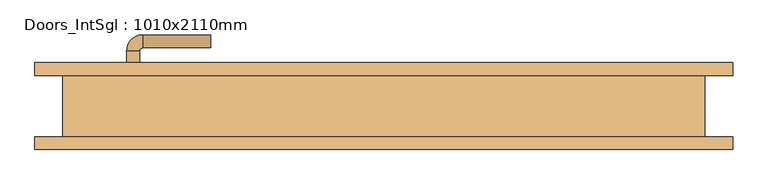
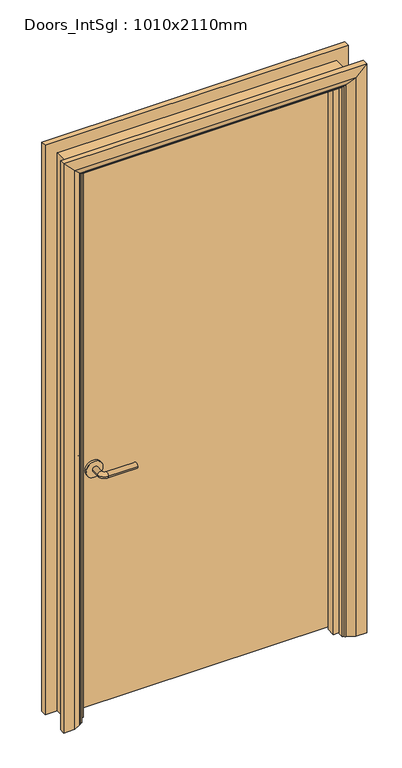
"""IFC4 building model written with IfcOpenShell, lengths in millimetres: door geometry, Doors_IntSgl : 1010x2110mm."""

import ifcopenshell
import ifcopenshell.guid

model = None  # the IFC model being written
_history = None  # IfcOwnerHistory: only IFC2X3 demands one
_inside = {}  # id of a spatial element -> (the spatial element, [elements in it])
_under = {}  # id of a project, library or spatial element -> (it, [spatial elements below it])
_declared = {}  # id of a project -> (the project, [libraries it declares])
_typed = {}  # id of a type object -> (the type object, [elements of that type])
_made_of = {}  # id of a material, layer set ... -> (it, [elements and type objects made of it])


def new_model(schema):
    """Start an empty IFC model of exactly this schema.

    Asked for "IFC4X3", IfcOpenShell would pick the latest addendum, in which some entities
    have other attributes; the version numbers below select the first issue.
    IFC2X3 requires an IfcOwnerHistory on every rooted entity: one is made here for all.
    """
    global model, _history
    if schema == "IFC4X3":
        model = ifcopenshell.file(schema_version=(4, 3, 0, 0))
    else:
        model = ifcopenshell.file(schema=schema)
    _inside.clear()
    _under.clear()
    _declared.clear()
    _typed.clear()
    _made_of.clear()
    _history = None
    if model.schema == "IFC2X3":
        org = make("IfcOrganization", Name="unknown")
        user = make(
            "IfcPersonAndOrganization",
            ThePerson=make("IfcPerson", FamilyName="unknown"),
            TheOrganization=org,
        )
        app = make(
            "IfcApplication",
            ApplicationDeveloper=org,
            Version="unknown",
            ApplicationFullName="unknown",
            ApplicationIdentifier="unknown",
        )
        _history = make(
            "IfcOwnerHistory",
            OwningUser=user,
            OwningApplication=app,
            ChangeAction="ADDED",
            CreationDate=0,
        )
    return model


def make(cls, **values):
    """One entity of the class cls with the attributes given. An attribute that is None is left unset."""
    return model.create_entity(
        cls, **{name: value for name, value in values.items() if value is not None}
    )


def rooted(cls, **values):
    """An entity with a GlobalId (a new one), such as an element, a storey or a relation."""
    return make(cls, GlobalId=ifcopenshell.guid.new(), OwnerHistory=_history, **values)


def si_unit(unit_type, name, prefix=None):
    """IfcSIUnit, for example si_unit("LENGTHUNIT", "METRE", prefix="MILLI")."""
    return make("IfcSIUnit", UnitType=unit_type, Prefix=prefix, Name=name)


def assignment(units):
    """IfcUnitAssignment: the units of a project."""
    return None if units is None else make("IfcUnitAssignment", Units=units)


def point(xyz):
    """IfcCartesianPoint."""
    return None if xyz is None else make("IfcCartesianPoint", Coordinates=xyz)


def direction(xyz):
    """IfcDirection."""
    return None if xyz is None else make("IfcDirection", DirectionRatios=xyz)


def frame(location, z_axis=None, x_axis=None):
    """IfcAxis2Placement3D, a coordinate frame: its origin and axes. An axis left out is left unset."""
    return make(
        "IfcAxis2Placement3D",
        Location=point(location),
        Axis=direction(z_axis),
        RefDirection=direction(x_axis),
    )


def frame_2d(location, x_axis=None):
    """IfcAxis2Placement2D, a coordinate frame in the plane: its origin and x axis."""
    return make(
        "IfcAxis2Placement2D", Location=point(location), RefDirection=direction(x_axis)
    )


def origin():
    """The frame at (0, 0, 0) with its axes left unset."""
    return frame((0.0, 0.0, 0.0))


def place(relative_to, where):
    """IfcLocalPlacement: puts the frame where relative to a parent placement (None: the world)."""
    return make(
        "IfcLocalPlacement", PlacementRelTo=relative_to, RelativePlacement=where
    )


def context(
    kind, dimensions, precision=None, world=None, true_north=None, identifier=None
):
    """IfcGeometricRepresentationContext, for example the 3D "Model" context."""
    return make(
        "IfcGeometricRepresentationContext",
        ContextIdentifier=identifier,
        ContextType=kind,
        CoordinateSpaceDimension=dimensions,
        Precision=precision,
        WorldCoordinateSystem=world,
        TrueNorth=true_north,
    )


def project(units=None, contexts=None):
    """IfcProject with its units and contexts."""
    return rooted(
        "IfcProject",
        Name="project",
        RepresentationContexts=contexts,
        UnitsInContext=assignment(units),
    )


def spatial(cls, under=None, at=None, **own):
    """A site, building, storey or space (cls), placed at a placement, below another one or the project."""
    s = rooted(cls, ObjectPlacement=at, **own)
    if under is not None:
        _under.setdefault(under.id(), (under, []))[1].append(s)
    return s


def polyline(points):
    """IfcPolyline through the points."""
    return make("IfcPolyline", Points=[point(p) for p in points])


def circle_curve(where, radius):
    """IfcCircle in the frame where."""
    return make("IfcCircle", Position=where, Radius=radius)


def ellipse_curve(where, semi_axis1, semi_axis2):
    """IfcEllipse in the frame where."""
    return make(
        "IfcEllipse", Position=where, SemiAxis1=semi_axis1, SemiAxis2=semi_axis2
    )


def trimmed(basis, trim1, trim2, sense, master):
    """IfcTrimmedCurve: the piece of a basis curve between two trims."""
    return make(
        "IfcTrimmedCurve",
        BasisCurve=basis,
        Trim1=trim1,
        Trim2=trim2,
        SenseAgreement=sense,
        MasterRepresentation=master,
    )


def segment(curve, same_sense, transition):
    """IfcCompositeCurveSegment."""
    return make(
        "IfcCompositeCurveSegment",
        Transition=transition,
        SameSense=same_sense,
        ParentCurve=curve,
    )


def composite_curve(segments, self_intersect=None):
    """IfcCompositeCurve: segments joined end to end."""
    return make("IfcCompositeCurve", Segments=segments, SelfIntersect=self_intersect)


def outline(outer, holes=None, kind="AREA"):
    """IfcArbitraryClosedProfileDef: a profile drawn as a closed curve; with holes, ...WithVoids."""
    if holes is None:
        return make("IfcArbitraryClosedProfileDef", ProfileType=kind, OuterCurve=outer)
    return make(
        "IfcArbitraryProfileDefWithVoids",
        ProfileType=kind,
        OuterCurve=outer,
        InnerCurves=holes,
    )


def extrude(swept, where, along, depth):
    """IfcExtrudedAreaSolid: the profile swept, set in the frame where, extruded along a direction by depth."""
    return make(
        "IfcExtrudedAreaSolid",
        SweptArea=swept,
        Position=where,
        ExtrudedDirection=direction(along),
        Depth=depth,
    )


def faces_of(points, faces, orient=None, outer=None):
    """IfcFace entities. A face is a list of loops; a loop is a list of indices into points, from 0.

    orient and outer hold one flag for each loop. By default every Orientation is true, the
    first loop of a face is its IfcFaceOuterBound and the others are IfcFaceBound.
    """
    made = []
    for i, loops in enumerate(faces):
        bounds = []
        for j, loop in enumerate(loops):
            is_outer = j == 0 if outer is None else outer[i][j]
            bounds.append(
                make(
                    "IfcFaceOuterBound" if is_outer else "IfcFaceBound",
                    Bound=make("IfcPolyLoop", Polygon=[points[k] for k in loop]),
                    Orientation=True if orient is None else orient[i][j],
                )
            )
        made.append(make("IfcFace", Bounds=bounds))
    return made


def faceted_brep(points, faces, orient=None, outer=None, voids=None):
    """IfcFacetedBrep: a solid bounded by flat faces; with voids (closed shells), ...WithVoids."""
    shared = [point(p) for p in points]
    hull = make("IfcClosedShell", CfsFaces=faces_of(shared, faces, orient, outer))
    if voids is None:
        return make("IfcFacetedBrep", Outer=hull)
    return make(
        "IfcFacetedBrepWithVoids",
        Outer=hull,
        Voids=[
            make(cls, CfsFaces=faces_of(shared, fs, o, b)) for cls, fs, o, b in voids
        ],
    )


def shape(context_of_items, identifier, shape_type, items):
    """IfcShapeRepresentation: the items that make up one representation, for example the "Body"."""
    return make(
        "IfcShapeRepresentation",
        ContextOfItems=context_of_items,
        RepresentationIdentifier=identifier,
        RepresentationType=shape_type,
        Items=items,
    )


def source(mapping_origin, context_of_items, identifier, shape_type, items):
    """IfcRepresentationMap: a shape defined once, which mapped items show again and again."""
    return make(
        "IfcRepresentationMap",
        MappingOrigin=mapping_origin,
        MappedRepresentation=shape(context_of_items, identifier, shape_type, items),
    )


def transform(
    local_origin,
    x_axis=None,
    y_axis=None,
    z_axis=None,
    scale=None,
    scale2=None,
    scale3=None,
    uniform=True,
):
    """IfcCartesianTransformationOperator3D, or its non-uniform kind. x_axis, y_axis, z_axis: its Axis1, 2, 3."""
    if uniform:
        return make(
            "IfcCartesianTransformationOperator3D",
            Axis1=direction(x_axis),
            Axis2=direction(y_axis),
            LocalOrigin=point(local_origin),
            Scale=scale,
            Axis3=direction(z_axis),
        )
    return make(
        "IfcCartesianTransformationOperator3DnonUniform",
        Axis1=direction(x_axis),
        Axis2=direction(y_axis),
        LocalOrigin=point(local_origin),
        Scale=scale,
        Axis3=direction(z_axis),
        Scale2=scale2,
        Scale3=scale3,
    )


def mapped(mapping_source, mapping_target):
    """IfcMappedItem: shows the shape of a source again, moved by a transform."""
    return make(
        "IfcMappedItem", MappingSource=mapping_source, MappingTarget=mapping_target
    )


def made_of(thing, what):
    """Note that an element or type object is made of a material, layer set ...; save() writes the relation."""
    if what is not None:
        _made_of.setdefault(what.id(), (what, []))[1].append(thing)
    return thing


def element(
    cls,
    number,
    at=None,
    inside=None,
    cuts=None,
    type_object=None,
    material=None,
    context=None,
    identifier="Body",
    shape_type=None,
    held_by="IfcProductDefinitionShape",
    body=None,
    shapes=None,
    **own,
):
    """One element of the class cls, such as IfcWall. Its Tag is "e" and its number.

    at: its placement. inside: the storey or other place that contains it. cuts: it is an
    opening in that element (IfcRelVoidsElement). A single representation is given by context,
    identifier, shape_type and body (its items); several are given by shapes. held_by: the class
    of the entity that holds the representations. save() writes the other relations.
    """
    e = rooted(cls, Tag="e%d" % number, ObjectPlacement=at, **own)
    if body is not None:
        shapes = [shape(context, identifier, shape_type, body)]
    if shapes is not None:
        e.Representation = make(held_by, Representations=shapes)
    if inside is not None:
        _inside.setdefault(inside.id(), (inside, []))[1].append(e)
    if cuts is not None:
        rooted(
            "IfcRelVoidsElement", RelatingBuildingElement=cuts, RelatedOpeningElement=e
        )
    if type_object is not None:
        _typed.setdefault(type_object.id(), (type_object, []))[1].append(e)
    return made_of(e, material)


def aggregate(whole, parts):
    """IfcRelAggregates: a whole, such as a stair, and the parts it consists of."""
    return rooted("IfcRelAggregates", RelatingObject=whole, RelatedObjects=parts)


def save(model, path):
    """Write the relations noted so far, then the file.

    IfcRelAggregates (storeys below a building ...), IfcRelContainedInSpatialStructure (elements
    in a storey), IfcRelDefinesByType, IfcRelAssociatesMaterial and IfcRelDeclares: one each for
    every whole, place, type object, material and project.
    """
    for whole, parts in _under.values():
        aggregate(whole, parts)
    for where, things in _inside.values():
        rooted(
            "IfcRelContainedInSpatialStructure",
            RelatedElements=things,
            RelatingStructure=where,
        )
    for kind, things in _typed.values():
        rooted("IfcRelDefinesByType", RelatedObjects=things, RelatingType=kind)
    for what, things in _made_of.values():
        rooted("IfcRelAssociatesMaterial", RelatedObjects=things, RelatingMaterial=what)
    for by, libraries in _declared.values():
        rooted("IfcRelDeclares", RelatingContext=by, RelatedDefinitions=libraries)
    model.write(path)


def plane_surface(at):
    """IfcPlane: the flat surface through the origin of the frame at, square to its z axis."""
    return make("IfcPlane", Position=at)


def cylinder_surface(at, radius):
    """IfcCylindricalSurface: all points at the distance radius from the z axis of the frame at."""
    return make("IfcCylindricalSurface", Position=at, Radius=radius)


def revolved_surface(curve, axis_point, axis_direction):
    """IfcSurfaceOfRevolution: the curve turned about the line through axis_point along axis_direction."""
    return make(
        "IfcSurfaceOfRevolution",
        SweptCurve=make("IfcArbitraryOpenProfileDef", ProfileType="CURVE", Curve=curve),
        AxisPosition=make("IfcAxis1Placement", Location=point(axis_point), Axis=direction(axis_direction)),
    )


def advanced_brep(points, edges, surfaces, faces):
    """IfcAdvancedBrep: a solid bounded by faces that lie on surfaces and meet in shared edges.

    An edge is (start, end): straight between two places in points (the first is 0);
    or (start, end, curve); or (start, end, curve, False) where it runs against its curve.
    A face is (place in surfaces, loops), or (place, loops, False) where it looks against
    its surface's normal. A loop lists edges by number (the first is 1), with a minus sign
    where the edge is run from its end to its start. The first loop is the outer one.
    """
    corners = [point(p) for p in points]
    vertices = [make("IfcVertexPoint", VertexGeometry=c) for c in corners]
    made = []
    for start, end, *more in edges:
        made.append(
            make(
                "IfcEdgeCurve",
                EdgeStart=vertices[start],
                EdgeEnd=vertices[end],
                EdgeGeometry=more[0] if more else make("IfcPolyline", Points=[corners[start], corners[end]]),
                SameSense=more[1] if len(more) > 1 else True,
            )
        )
    hull = []
    for where, loops, *sense in faces:
        bounds = []
        for j, loop in enumerate(loops):
            ring = [make("IfcOrientedEdge", EdgeElement=made[abs(k) - 1], Orientation=k > 0) for k in loop]
            bounds.append(
                make(
                    "IfcFaceOuterBound" if j == 0 else "IfcFaceBound",
                    Bound=make("IfcEdgeLoop", EdgeList=ring),
                    Orientation=True,
                )
            )
        hull.append(make("IfcAdvancedFace", Bounds=bounds, FaceSurface=surfaces[where], SameSense=sense[0] if sense else True))
    return make("IfcAdvancedBrep", Outer=make("IfcClosedShell", CfsFaces=hull))


def doors_intsgl_1010x2110mm_9b3ab836(model_context):
    return source(origin(), model_context, "Body", "SolidModel", [
        advanced_brep(
        [(-398.0, 1.5, 900.0), (-378.0, 1.5, 900.0), (-378.0, -28.5, 900.0), (-398.0, -28.5, 900.0), (-373.0, -33.5, 900.0), (-373.0, -53.5, 900.0), (-268.0, -53.5, 900.0), (-268.0, -33.5, 900.0)],
        [
            (0, 1, circle_curve(frame((-388.0, 1.5, 900.0), z_axis=(0.0, 1.0, 0.0), x_axis=(1.0, 0.0, 0.0)), 10.0)),
            (1, 0, circle_curve(frame((-388.0, 1.5, 900.0), z_axis=(0.0, 1.0, 0.0), x_axis=(1.0, 0.0, 0.0)), 10.0)),
            (1, 2),
            (2, 3, circle_curve(frame((-388.0, -28.5, 900.0), z_axis=(0.0, 1.0, 0.0), x_axis=(1.0, 0.0, 0.0)), 10.0)),
            (3, 0),
            (3, 2, circle_curve(frame((-388.0, -28.5, 900.0), z_axis=(0.0, 1.0, 0.0), x_axis=(1.0, 0.0, 0.0)), 10.0)),
            (4, 5, circle_curve(frame((-373.0, -43.5, 900.0), z_axis=(-1.0, 0.0, 0.0), x_axis=(0.0, 1.0, 0.0)), 10.0)),
            (5, 3, circle_curve(frame((-373.0, -28.5, 900.0), z_axis=(0.0, 0.0, -1.0), x_axis=(-1.0, 0.0, 0.0)), 25.0)),
            (2, 4, circle_curve(frame((-373.0, -28.5, 900.0), z_axis=(0.0, 0.0, 1.0), x_axis=(-1.0, 0.0, 0.0)), 5.0)),
            (5, 4, circle_curve(frame((-373.0, -43.5, 900.0), z_axis=(-1.0, 0.0, 0.0), x_axis=(0.0, 1.0, 0.0)), 10.0)),
            (6, 7, circle_curve(frame((-268.0, -43.5, 900.0), z_axis=(1.0, 0.0, 0.0), x_axis=(0.0, 1.0, 0.0)), 10.0)),
            (7, 6, circle_curve(frame((-268.0, -43.5, 900.0), z_axis=(1.0, 0.0, 0.0), x_axis=(0.0, 1.0, 0.0)), 10.0)),
            (4, 7),
            (6, 5),
        ],
        [
            plane_surface(frame((-388.0, 1.5, 900.0), z_axis=(0.0, 1.0, 0.0), x_axis=(0.0, 0.0, 1.0))),
            cylinder_surface(frame((-388.0, 1.5, 900.0), z_axis=(0.0, 1.0, 0.0), x_axis=(1.0, 0.0, 0.0)), 10.0),
            revolved_surface(trimmed(ellipse_curve(frame((-388.0, -28.5, 900.0), z_axis=(0.0, -1.0, 0.0), x_axis=(1.0, 0.0, 0.0)), 10.0, 10.0), [point((-398.0, -28.5, 900.0))], [point((-378.0, -28.5, 900.0))], True, "CARTESIAN"), (-373.0, -28.5, 900.0), (0.0, 0.0, -1.0)),
            revolved_surface(trimmed(ellipse_curve(frame((-388.0, -28.5, 900.0), z_axis=(0.0, -1.0, 0.0), x_axis=(1.0, 0.0, 0.0)), 10.0, 10.0), [point((-378.0, -28.5, 900.0))], [point((-398.0, -28.5, 900.0))], True, "CARTESIAN"), (-373.0, -28.5, 900.0), (0.0, 0.0, -1.0)),
            plane_surface(frame((-268.0, -43.5, 900.0), z_axis=(1.0, 0.0, 0.0), x_axis=(0.0, 0.0, 1.0))),
            cylinder_surface(frame((-373.0, -43.5, 900.0), z_axis=(-1.0, 0.0, 0.0), x_axis=(0.0, 1.0, 0.0)), 10.0),
        ],
        [
            (0, [[1, 2]]),
            (1, [[3, 4, 5, -2]]),
            (1, [[-5, 6, -3, -1]]),
            (2, [[7, 8, -4, 9]]),
            (3, [[10, -9, -6, -8]]),
            (4, [[11, 12]]),
            (5, [[13, -11, 14, -7]]),
            (5, [[-14, -12, -13, -10]]),
        ],
    ),
        extrude(outline(composite_curve([segment(trimmed(circle_curve(frame_2d((900.0, -390.5)), 30.0), [point((900.0, -420.5))], [point((900.0, -360.5))], False, "CARTESIAN"), True, "CONTINUOUS"), segment(trimmed(circle_curve(frame_2d((900.0, -390.5)), 30.0), [point((900.0, -360.5))], [point((900.0, -420.5))], False, "CARTESIAN"), True, "CONTINUOUS")], self_intersect=False)), frame((0.0, 1.5, 0.0), z_axis=(0.0, 1.0, 0.0), x_axis=(0.0, 0.0, 1.0)), (0.0, 0.0, 1.0), 8.0),
        advanced_brep(
        [(-398.0, 55.5, 900.0), (-378.0, 55.5, 900.0), (-398.0, 85.5, 900.0), (-378.0, 85.5, 900.0), (-373.0, 90.5, 900.0), (-373.0, 110.5, 900.0), (-268.0, 110.5, 900.0), (-268.0, 90.5, 900.0)],
        [
            (0, 1, circle_curve(frame((-388.0, 55.5, 900.0), z_axis=(0.0, -1.0, 0.0), x_axis=(1.0, 0.0, 0.0)), 10.0)),
            (1, 0, circle_curve(frame((-388.0, 55.5, 900.0), z_axis=(0.0, -1.0, 0.0), x_axis=(1.0, 0.0, 0.0)), 10.0)),
            (0, 2),
            (2, 3, circle_curve(frame((-388.0, 85.5, 900.0), z_axis=(0.0, -1.0, 0.0), x_axis=(1.0, 0.0, 0.0)), 10.0)),
            (3, 1),
            (3, 2, circle_curve(frame((-388.0, 85.5, 900.0), z_axis=(0.0, -1.0, 0.0), x_axis=(1.0, 0.0, 0.0)), 10.0)),
            (4, 3, circle_curve(frame((-373.0, 85.5, 900.0), z_axis=(0.0, 0.0, 1.0), x_axis=(-1.0, 0.0, 0.0)), 5.0)),
            (2, 5, circle_curve(frame((-373.0, 85.5, 900.0), z_axis=(0.0, 0.0, -1.0), x_axis=(-1.0, 0.0, 0.0)), 25.0)),
            (5, 4, circle_curve(frame((-373.0, 100.5, 900.0), z_axis=(-1.0, 0.0, 0.0), x_axis=(0.0, -1.0, 0.0)), 10.0)),
            (4, 5, circle_curve(frame((-373.0, 100.5, 900.0), z_axis=(-1.0, 0.0, 0.0), x_axis=(0.0, -1.0, 0.0)), 10.0)),
            (6, 7, circle_curve(frame((-268.0, 100.5, 900.0), z_axis=(1.0, 0.0, 0.0), x_axis=(0.0, -1.0, 0.0)), 10.0)),
            (7, 6, circle_curve(frame((-268.0, 100.5, 900.0), z_axis=(1.0, 0.0, 0.0), x_axis=(0.0, -1.0, 0.0)), 10.0)),
            (5, 6),
            (7, 4),
        ],
        [
            plane_surface(frame((-388.0, 55.5, 900.0), z_axis=(0.0, -1.0, 0.0), x_axis=(0.0, 0.0, 1.0))),
            cylinder_surface(frame((-388.0, 55.5, 900.0), z_axis=(0.0, -1.0, 0.0), x_axis=(1.0, 0.0, 0.0)), 10.0),
            revolved_surface(trimmed(ellipse_curve(frame((-388.0, 85.5, 900.0), z_axis=(0.0, -1.0, 0.0), x_axis=(1.0, 0.0, 0.0)), 10.0, 10.0), [point((-398.0, 85.5, 900.0))], [point((-378.0, 85.5, 900.0))], True, "CARTESIAN"), (-373.0, 85.5, 900.0), (0.0, 0.0, -1.0)),
            revolved_surface(trimmed(ellipse_curve(frame((-388.0, 85.5, 900.0), z_axis=(0.0, -1.0, 0.0), x_axis=(1.0, 0.0, 0.0)), 10.0, 10.0), [point((-378.0, 85.5, 900.0))], [point((-398.0, 85.5, 900.0))], True, "CARTESIAN"), (-373.0, 85.5, 900.0), (0.0, 0.0, -1.0)),
            plane_surface(frame((-268.0, 100.5, 900.0), z_axis=(1.0, 0.0, 0.0), x_axis=(0.0, 0.0, 1.0))),
            cylinder_surface(frame((-373.0, 100.5, 900.0), z_axis=(-1.0, 0.0, 0.0), x_axis=(0.0, -1.0, 0.0)), 10.0),
        ],
        [
            (0, [[1, 2]]),
            (1, [[-1, 3, 4, 5]]),
            (1, [[-2, -5, 6, -3]]),
            (2, [[7, -4, 8, 9]]),
            (3, [[-8, -6, -7, 10]]),
            (4, [[11, 12]]),
            (5, [[-9, 13, -12, 14]]),
            (5, [[-10, -14, -11, -13]]),
        ],
    ),
        extrude(outline(composite_curve([segment(trimmed(circle_curve(frame_2d((900.0, -390.5)), 30.0), [point((900.0, -420.5))], [point((900.0, -360.5))], False, "CARTESIAN"), True, "CONTINUOUS"), segment(trimmed(circle_curve(frame_2d((900.0, -390.5)), 30.0), [point((900.0, -360.5))], [point((900.0, -420.5))], False, "CARTESIAN"), True, "CONTINUOUS")], self_intersect=False)), frame((0.0, 47.5, 0.0), z_axis=(0.0, 1.0, 0.0), x_axis=(0.0, 0.0, 1.0)), (0.0, 0.0, 1.0), 8.0),
        extrude(outline(polyline([(463.0, 9.5), (-463.0, 9.5), (-463.0, 47.5), (463.0, 47.5), (463.0, 9.5)])), frame((0.0, 0.0, 8.0), z_axis=(0.0, 0.0, 1.0), x_axis=(1.0, 0.0, 0.0)), (0.0, 0.0, 1.0), 2060.0),
        advanced_brep(
        [(540.0, 67.5, 0.0), (540.0, 47.5, 0.0), (470.0, 47.5, 0.0), (474.0, 53.5, 0.0), (500.0, 67.5, 0.0), (540.0, 67.5, 2145.0), (540.0, 47.5, 2145.0), (-540.0, 47.5, 2145.0), (-540.0, 47.5, 0.0), (-470.0, 47.5, 0.0), (-470.0, 47.5, 2075.0), (470.0, 47.5, 2075.0), (474.0, 53.5, 2079.0), (500.0, 67.5, 2105.0), (-500.0, 67.5, 2105.0), (-500.0, 67.5, 0.0), (-540.0, 67.5, 0.0), (-540.0, 67.5, 2145.0), (-474.0, 53.5, 2079.0), (-474.0, 53.5, 0.0)],
        [
            (0, 1),
            (1, 2),
            (2, 3, circle_curve(frame((478.0, 46.5, 0.0), z_axis=(0.0, 0.0, -1.0), x_axis=(1.0, 0.0, 0.0)), 8.0622577)),
            (3, 4),
            (4, 0),
            (0, 5),
            (5, 6),
            (6, 1),
            (6, 7),
            (7, 8),
            (8, 9),
            (9, 10),
            (10, 11),
            (11, 2),
            (11, 12, ellipse_curve(frame((478.0, 46.5, 2083.0), z_axis=(0.7071067811865475, 0.0, -0.7071067811865475), x_axis=(-0.7071067811865474, 0.0, -0.7071067811865476)), 11.4017543, 8.0622577)),
            (12, 3),
            (12, 13),
            (13, 4),
            (13, 14),
            (14, 15),
            (15, 16),
            (16, 17),
            (17, 5),
            (17, 7),
            (10, 18, ellipse_curve(frame((-478.0, 46.5, 2083.0), z_axis=(0.7071067811865475, 0.0, 0.7071067811865475), x_axis=(0.7071067811865476, 0.0, -0.7071067811865474)), 11.4017543, 8.0622577)),
            (18, 12),
            (18, 14),
            (15, 19),
            (19, 9, circle_curve(frame((-478.0, 46.5, 0.0), z_axis=(0.0, 0.0, -1.0), x_axis=(-1.0, 0.0, 0.0)), 8.0622577)),
            (8, 16),
            (19, 18),
        ],
        [
            plane_surface(frame((470.0, 47.5, 0.0), z_axis=(0.0, 0.0, -1.0), x_axis=(0.0, -1.0, 0.0))),
            plane_surface(frame((540.0, 67.5, 0.0), z_axis=(1.0, 0.0, 0.0), x_axis=(0.0, 0.0, 1.0))),
            plane_surface(frame((540.0, 47.5, 0.0), z_axis=(0.0, -1.0, 0.0), x_axis=(0.0, 0.0, 1.0))),
            cylinder_surface(frame((478.0, 46.5, 0.0), z_axis=(0.0, 0.0, -1.0), x_axis=(1.0, 0.0, 0.0)), 8.0622577),
            plane_surface(frame((474.0, 53.5, 0.0), z_axis=(-0.4740998230350126, 0.880471099922178, 0.0), x_axis=(0.0, 0.0, 1.0))),
            plane_surface(frame((500.0, 67.5, 0.0), z_axis=(0.0, 1.0, 0.0), x_axis=(0.0, 0.0, 1.0))),
            plane_surface(frame((540.0, 67.5, 2145.0), z_axis=(0.0, 0.0, 1.0), x_axis=(-1.0, 0.0, 0.0))),
            cylinder_surface(frame((470.0, 46.5, 2083.0), z_axis=(1.0, 0.0, 0.0), x_axis=(0.0, 0.0, 1.0)), 8.0622577),
            plane_surface(frame((474.0, 53.5, 2079.0), z_axis=(0.0, 0.8804710999221764, -0.4740998230350154), x_axis=(-1.0, 0.0, 0.0))),
            plane_surface(frame((-470.0, 47.5, 0.0), z_axis=(0.0, 0.0, -1.0), x_axis=(0.0, -1.0, 0.0))),
            plane_surface(frame((-540.0, 67.5, 2145.0), z_axis=(-1.0, 0.0, 0.0), x_axis=(0.0, 0.0, -1.0))),
            cylinder_surface(frame((-478.0, 46.5, 2075.0), z_axis=(0.0, 0.0, 1.0), x_axis=(-1.0, 0.0, 0.0)), 8.0622577),
            plane_surface(frame((-474.0, 53.5, 2079.0), z_axis=(0.47409982303501824, 0.8804710999221749, 0.0), x_axis=(0.0, 0.0, -1.0))),
        ],
        [
            (0, [[1, 2, 3, 4, 5]]),
            (1, [[-1, 6, 7, 8]]),
            (2, [[-2, -8, 9, 10, 11, 12, 13, 14]]),
            (3, [[-3, -14, 15, 16]]),
            (4, [[-4, -16, 17, 18]]),
            (5, [[-5, -18, 19, 20, 21, 22, 23, -6]]),
            (6, [[-7, -23, 24, -9]]),
            (7, [[-15, -13, 25, 26]]),
            (8, [[-17, -26, 27, -19]]),
            (9, [[-21, 28, 29, -11, 30]]),
            (10, [[-24, -22, -30, -10]]),
            (11, [[-25, -12, -29, 31]]),
            (12, [[-27, -31, -28, -20]]),
        ],
    ),
        extrude(outline(polyline([(0.0, -465.0), (0.0, -446.0), (2051.0, -446.0), (2051.0, 446.0), (0.0, 446.0), (0.0, 465.0), (2070.0, 465.0), (2070.0, -465.0), (0.0, -465.0)])), frame((0.0, -24.5, 0.0), z_axis=(0.0, 1.0, 0.0), x_axis=(0.0, 0.0, 1.0)), (0.0, 0.0, 1.0), 32.0),
        advanced_brep(
        [(-540.0, -67.5, 0.0), (-540.0, -47.5, 0.0), (-470.0, -47.5, 0.0), (-474.0, -53.5, 0.0), (-500.0, -67.5, 0.0), (-540.0, -67.5, 2145.0), (-540.0, -47.5, 2145.0), (-470.0, -47.5, 2075.0), (-474.0, -53.5, 2079.0), (-500.0, -67.5, 2105.0), (540.0, -67.5, 2145.0), (540.0, -47.5, 2145.0), (470.0, -47.5, 2075.0), (474.0, -53.5, 2079.0), (500.0, -67.5, 2105.0), (540.0, -67.5, 0.0), (500.0, -67.5, 0.0), (474.0, -53.5, 0.0), (470.0, -47.5, 0.0), (540.0, -47.5, 0.0)],
        [
            (0, 1),
            (1, 2),
            (2, 3, circle_curve(frame((-478.0, -46.5, 0.0), z_axis=(0.0, 0.0, -1.0), x_axis=(-1.0, 0.0, 0.0)), 8.0622577)),
            (3, 4),
            (4, 0),
            (0, 5),
            (5, 6),
            (6, 1),
            (6, 7),
            (7, 2),
            (7, 8, ellipse_curve(frame((-478.0, -46.5, 2083.0), z_axis=(-0.7071067811865475, 0.0, -0.7071067811865475), x_axis=(0.7071067811865474, 0.0, -0.7071067811865476)), 11.4017543, 8.0622577)),
            (8, 3),
            (8, 9),
            (9, 4),
            (9, 5),
            (5, 10),
            (10, 11),
            (11, 6),
            (11, 12),
            (12, 7),
            (12, 13, ellipse_curve(frame((478.0, -46.5, 2083.0), z_axis=(-0.7071067811865475, 0.0, 0.7071067811865475), x_axis=(-0.7071067811865476, 0.0, -0.7071067811865474)), 11.4017543, 8.0622577)),
            (13, 8),
            (13, 14),
            (14, 9),
            (14, 10),
            (15, 16),
            (16, 17),
            (17, 18, circle_curve(frame((478.0, -46.5, 0.0), z_axis=(0.0, 0.0, -1.0), x_axis=(1.0, 0.0, 0.0)), 8.0622577)),
            (18, 19),
            (19, 15),
            (10, 15),
            (19, 11),
            (18, 12),
            (17, 13),
            (16, 14),
        ],
        [
            plane_surface(frame((-470.0, -120.3010989, 0.0), z_axis=(0.0, 0.0, -1.0), x_axis=(1.0, 0.0, 0.0))),
            plane_surface(frame((-540.0, -67.5, 0.0), z_axis=(-1.0, 0.0, 0.0), x_axis=(0.0, 0.0, 1.0))),
            plane_surface(frame((-540.0, -47.5, 0.0), z_axis=(0.0, 1.0, 0.0), x_axis=(0.0, 0.0, 1.0))),
            cylinder_surface(frame((-478.0, -46.5, 0.0), z_axis=(0.0, 0.0, -1.0), x_axis=(-1.0, 0.0, 0.0)), 8.0622577),
            plane_surface(frame((-474.0, -53.5, 0.0), z_axis=(0.4740998230350183, -0.8804710999221749, 0.0), x_axis=(0.0, 0.0, 1.0))),
            plane_surface(frame((-500.0, -67.5, 0.0), z_axis=(0.0, -1.0, 0.0), x_axis=(0.0, 0.0, 1.0))),
            plane_surface(frame((-540.0, -67.5, 2145.0), z_axis=(0.0, 0.0, 1.0), x_axis=(1.0, 0.0, 0.0))),
            plane_surface(frame((-540.0, -47.5, 2145.0), z_axis=(0.0, 1.0, 0.0), x_axis=(1.0, 0.0, 0.0))),
            cylinder_surface(frame((-470.0, -46.5, 2083.0), z_axis=(-1.0, 0.0, 0.0), x_axis=(0.0, 0.0, 1.0)), 8.0622577),
            plane_surface(frame((-474.0, -53.5, 2079.0), z_axis=(0.0, -0.8804710999221749, -0.4740998230350183), x_axis=(1.0, 0.0, 0.0))),
            plane_surface(frame((-500.0, -67.5, 2105.0), z_axis=(0.0, -1.0, 0.0), x_axis=(1.0, 0.0, 0.0))),
            plane_surface(frame((470.0, -120.3010989, 0.0), z_axis=(0.0, 0.0, -1.0), x_axis=(-1.0, 0.0, 0.0))),
            plane_surface(frame((540.0, -67.5, 2145.0), z_axis=(1.0, 0.0, 0.0), x_axis=(0.0, 0.0, -1.0))),
            plane_surface(frame((540.0, -47.5, 2145.0), z_axis=(0.0, 1.0, 0.0), x_axis=(0.0, 0.0, -1.0))),
            cylinder_surface(frame((478.0, -46.5, 2075.0), z_axis=(0.0, 0.0, 1.0), x_axis=(1.0, 0.0, 0.0)), 8.0622577),
            plane_surface(frame((474.0, -53.5, 2079.0), z_axis=(-0.4740998230350183, -0.8804710999221749, 0.0), x_axis=(0.0, 0.0, -1.0))),
            plane_surface(frame((500.0, -67.5, 2105.0), z_axis=(0.0, -1.0, 0.0), x_axis=(0.0, 0.0, -1.0))),
        ],
        [
            (0, [[1, 2, 3, 4, 5]]),
            (1, [[-1, 6, 7, 8]]),
            (2, [[-2, -8, 9, 10]]),
            (3, [[-3, -10, 11, 12]]),
            (4, [[-4, -12, 13, 14]]),
            (5, [[-5, -14, 15, -6]]),
            (6, [[-7, 16, 17, 18]]),
            (7, [[-9, -18, 19, 20]]),
            (8, [[-11, -20, 21, 22]]),
            (9, [[-13, -22, 23, 24]]),
            (10, [[-15, -24, 25, -16]]),
            (11, [[26, 27, 28, 29, 30]]),
            (12, [[-17, 31, -30, 32]]),
            (13, [[-19, -32, -29, 33]]),
            (14, [[-21, -33, -28, 34]]),
            (15, [[-23, -34, -27, 35]]),
            (16, [[-25, -35, -26, -31]]),
        ],
    ),
        faceted_brep([(-465.0, 47.5, 0.0), (-465.0, -47.5, 0.0), (-497.0, -47.5, 0.0), (-497.0, 47.5, 0.0), (-465.0, 47.5, 2070.0), (-465.0, -47.5, 2070.0), (-497.0, -47.5, 2102.0), (-497.0, 47.5, 2102.0), (465.0, 47.5, 2070.0), (465.0, -47.5, 2070.0), (497.0, -47.5, 2102.0), (497.0, 47.5, 2102.0), (465.0, 47.5, 0.0), (497.0, 47.5, 0.0), (497.0, -47.5, 0.0), (465.0, -47.5, 0.0)], [[[0, 1, 2, 3]], [[1, 0, 4, 5]], [[2, 1, 5, 6]], [[3, 2, 6, 7]], [[0, 3, 7, 4]], [[5, 4, 8, 9]], [[6, 5, 9, 10]], [[7, 6, 10, 11]], [[4, 7, 11, 8]], [[12, 13, 14, 15]], [[9, 8, 12, 15]], [[10, 9, 15, 14]], [[11, 10, 14, 13]], [[8, 11, 13, 12]]]),
    ])


if __name__ == "__main__":
    model = new_model("IFC4")
    model_context = context("Model", 3, world=origin())
    ifc_project = project(units=[si_unit("LENGTHUNIT", "METRE", prefix="MILLI")], contexts=[model_context])
    site = spatial("IfcSite", under=ifc_project)
    building = spatial("IfcBuilding", under=site)
    placement = place(None, origin())
    doors_intsgl_1010x2110mm_shape = doors_intsgl_1010x2110mm_9b3ab836(model_context)
    element("IfcDoor", 1, ObjectType="Doors_IntSgl : 1010x2110mm", at=placement, inside=building, context=model_context, shape_type="MappedRepresentation", body=[
        mapped(doors_intsgl_1010x2110mm_shape, transform((0.0, 0.0, 0.0), x_axis=(1.0, 0.0, 0.0), y_axis=(0.0, 1.0, 0.0), z_axis=(0.0, 0.0, 1.0))),
    ])
    save(model, "model.ifc")

# Revit data of these elements
# Type "Doors_IntSgl : 1010x2110mm"
#   Construction Type Id = "MDOOR"
#   Type Mark = "43"
#   Type Comments = "Internal Single"
#   Operation = "SingleSwingRight"
#   Manufacturer = "Revit"
#   Keynote = "L20"
#   Description = "Internal Single Door"
#   Analytic Construction = "Metal"
#   UnderCut = 8 mm
#   Tolerance = 2 mm
#   Thickness = 38 mm
#   Thermal Resistance (R) = 0.270117 (m²·K)/W
#   Structural Tolerance = 8 mm
#   StopDepth = 32 mm
#   Stop Thickness = 19 mm
#   Rough Width = 1010 mm
#   Rough Height = 2110 mm
#   Height to Top Lock Rail = 1000 mm
#   Heat Transfer Coefficient (U) = 3.7021 W/(m²·K)
#   Handle Z Distance = 900 mm
#   Handle X Distance = 75 mm
#   Frame Thickness = 32 mm
#   Door Panel Width = 926 mm
#   Door Panel Thickness = 38 mm
#   Door Panel Offset = 0 mm
#   Height = 2110 mm
#   Width = 1010 mm
#   Door Panel Height = 2060 mm
#   Architrave Setback = 5 mm
#   Vis - Ironmongery = yes
#   Material Ironmongery = Door - Handle
#   Material Frame = Door - Frame/Mullion (1)
#   Material Door = Door - Panel
#   Material Architrave = Door - Architrave
#   Visual Light Transmittance = 0
#   Solar Heat Gain Coefficient = 0
#   Function = (empty or 0)
#   Wall Closure = (empty or 0)
# Element 1 (IfcDoor, "Doors_IntSgl : 1010x2110mm")
#   Materials on its faces: "Door - Architrave", "Door - Handle", "Door - Frame/Mullion (1)", "Door - Panel"
# Materials
#   "Door - Handle": class "Miscellaneous", colour RGB 0 0 0, transparency 0, Keynote = "P21", Cost = 0
#   "Door - Frame/Mullion (1)": class "Wood", colour RGB 212 179 113, transparency 0, Keynote = "L20", Cost = 0
#   "Door - Panel": class "Wood", colour RGB 210 159 95, transparency 0, Keynote = "L20", Cost = 0
#   "Door - Architrave": class "Wood", colour RGB 154 90 5, transparency 0, Keynote = "P20", Cost = 0
